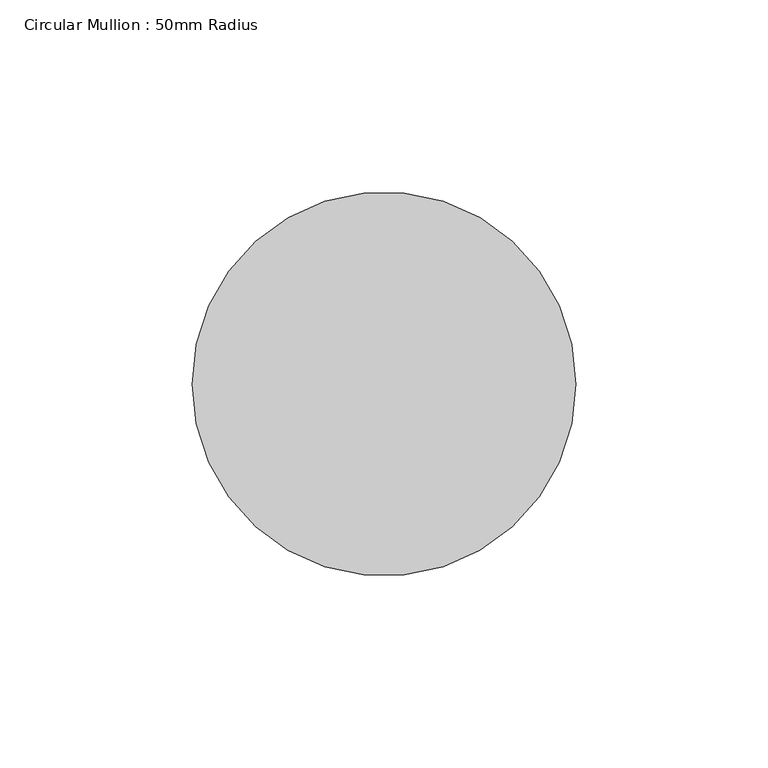
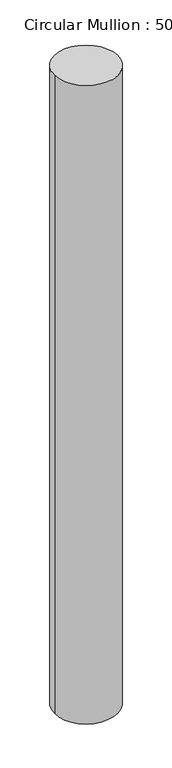
"""IFC4 building model written with IfcOpenShell, lengths in millimetres: member geometry, Circular Mullion : 50mm Radius."""

from ifc_helpers import new_model, si_unit, frame, origin, place, context, project, spatial, ellipse_curve, source, transform, mapped, element, save
from ifc_brep_helpers import plane_surface, cylinder_surface, advanced_brep


def circular_mullion_50mm_radius_174610fd(model_context):
    return source(origin(), model_context, "Body", "AdvancedBrep", [
        advanced_brep(
        [(-100.0, 0.0, 1.2595412), (0.0, 0.0, 0.0), (0.0, 0.0, -1068.5203263), (-100.0, 0.0, -1069.8156922)],
        [
            (0, 1, ellipse_curve(frame((-50.0, 0.0, 0.6297706), z_axis=(-0.012592959485159932, -0.015193000350894076, -0.9998052760971723), x_axis=(-0.6380280065478242, -0.7697602568152971, 0.019733471267291657)), 50.0097381, 50.0)),
            (1, 2),
            (2, 3, ellipse_curve(frame((-50.0, 0.0, -1069.1680092), z_axis=(-0.012950991534684866, -0.01562495449641879, 0.9997940450989162), x_axis=(0.6380208394608387, 0.7697516099554069, 0.020294516124952686)), 50.0102999, 50.0)),
            (3, 0),
            (1, 0, ellipse_curve(frame((-50.0, 0.0, 0.6297706), z_axis=(-0.012592959485159932, -0.015193000350894076, -0.9998052760971723), x_axis=(-0.6380280065478242, -0.7697602568152971, 0.019733471267291657)), 50.0097381, 50.0)),
            (3, 2, ellipse_curve(frame((-50.0, 0.0, -1069.1680092), z_axis=(-0.012950991534684866, -0.01562495449641879, 0.9997940450989162), x_axis=(0.6380208394608387, 0.7697516099554069, 0.020294516124952686)), 50.0102999, 50.0)),
        ],
        [
            cylinder_surface(frame((-50.0, 0.0, 0.0), z_axis=(0.0, 0.0, 1.0), x_axis=(1.0, 0.0, 0.0)), 50.0),
            plane_surface(frame((-234.6686219, 194.5088119, 0.0), z_axis=(0.012592959485159936, 0.01519300035089408, 0.9998052760971725), x_axis=(0.6380280065478241, 0.7697602568152975, -0.01973347126729474))),
            plane_surface(frame((-234.6686219, 194.5088119, -1068.5203263), z_axis=(0.012950991534684863, 0.015624954496418786, -0.999794045098916), x_axis=(0.6380208394608383, 0.7697516099554067, 0.020294516124969242))),
        ],
        [
            (0, [[1, 2, 3, 4]]),
            (0, [[5, -4, 6, -2]]),
            (1, [[-1, -5]]),
            (2, [[-6, -3]]),
        ],
    ),
    ])


if __name__ == "__main__":
    model = new_model("IFC4")
    model_context = context("Model", 3, world=origin())
    ifc_project = project(units=[si_unit("LENGTHUNIT", "METRE", prefix="MILLI")], contexts=[model_context])
    site = spatial("IfcSite", under=ifc_project)
    building = spatial("IfcBuilding", under=site)
    placement = place(None, origin())
    circular_mullion_50mm_radius_shape = circular_mullion_50mm_radius_174610fd(model_context)
    element("IfcMember", 1, ObjectType="Circular Mullion : 50mm Radius", at=placement, inside=building, context=model_context, shape_type="MappedRepresentation", body=[
        mapped(circular_mullion_50mm_radius_shape, transform((0.0, 0.0, 0.0), x_axis=(1.0, 0.0, 0.0), y_axis=(0.0, 1.0, 0.0), z_axis=(0.0, 0.0, 1.0))),
    ])
    save(model, "model.ifc")

# Revit data of these elements
# Type "Circular Mullion : 50mm Radius"
#   built-in parameter 1007350 = 0.164042 (stored number, unit not read)
# Element 1 (IfcMember, "Circular Mullion : 50mm Radius")
#   Materials on its faces: "Aluminium"
# Materials
#   "Aluminium": class "Metal", colour RGB 247 247 247, transparency 0, Description = "Aluminium 6061", Cost = 0
